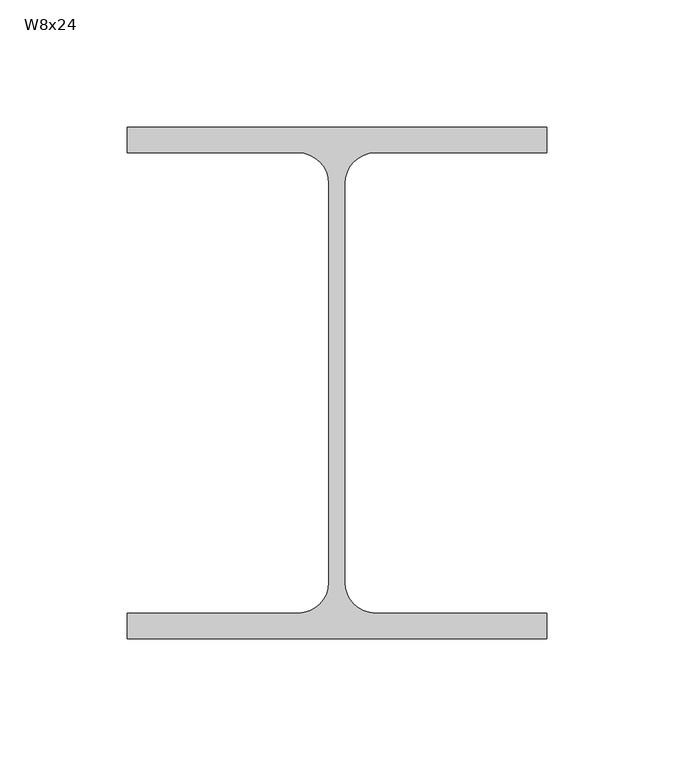
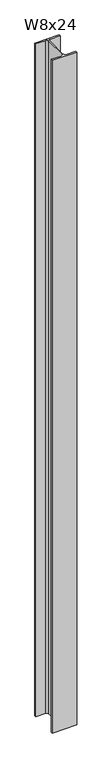
"""IFC4 building model written with IfcOpenShell, lengths in millimetres: column geometry, RME WF - Column : W8x24."""

from ifc_helpers import new_model, si_unit, point, frame, frame_2d, origin, place, context, project, spatial, polyline, circle_curve, trimmed, segment, composite_curve, outline, extrude, source, transform, mapped, element, save


def w8x24_d83c1f9c(model_context):
    return source(origin(), model_context, "Body", "SweptSolid", [
        extrude(outline(composite_curve([segment(polyline([(82.55, 100.711), (82.55, 90.551), (15.1765, 90.551)]), True, "CONTINUOUS"), segment(trimmed(circle_curve(frame_2d((15.1765, 78.486)), 12.065), [point((15.1765, 90.551))], [point((3.1115, 78.486))], True, "CARTESIAN"), True, "CONTINUOUS"), segment(polyline([(3.1115, 78.486), (3.1115, -78.486)]), True, "CONTINUOUS"), segment(trimmed(circle_curve(frame_2d((15.1765, -78.486)), 12.065), [point((3.1115, -78.486))], [point((15.1765, -90.551))], True, "CARTESIAN"), True, "CONTINUOUS"), segment(polyline([(15.1765, -90.551), (82.55, -90.551), (82.55, -100.711), (-82.55, -100.711), (-82.55, -90.551), (-15.1765, -90.551)]), True, "CONTINUOUS"), segment(trimmed(circle_curve(frame_2d((-15.1765, -78.486)), 12.065), [point((-15.1765, -90.551))], [point((-3.1115, -78.486))], True, "CARTESIAN"), True, "CONTINUOUS"), segment(polyline([(-3.1115, -78.486), (-3.1115, 78.486)]), True, "CONTINUOUS"), segment(trimmed(circle_curve(frame_2d((-15.1765, 78.486)), 12.065), [point((-3.1115, 78.486))], [point((-15.1765, 90.551))], True, "CARTESIAN"), True, "CONTINUOUS"), segment(polyline([(-15.1765, 90.551), (-82.55, 90.551), (-82.55, 100.711), (82.55, 100.711)]), True, "CONTINUOUS")], self_intersect=False)), frame((0.0, 0.0, -304.8), z_axis=(0.0, 0.0, 1.0), x_axis=(1.0, 0.0, 0.0)), (0.0, 0.0, 1.0), 4791.075),
    ])


if __name__ == "__main__":
    model = new_model("IFC4")
    model_context = context("Model", 3, world=origin())
    ifc_project = project(units=[si_unit("LENGTHUNIT", "METRE", prefix="MILLI")], contexts=[model_context])
    site = spatial("IfcSite", under=ifc_project)
    building = spatial("IfcBuilding", under=site)
    placement = place(None, origin())
    w8x24_shape = w8x24_d83c1f9c(model_context)
    element("IfcColumn", 1, ObjectType="RME WF - Column : W8x24", at=placement, inside=building, context=model_context, shape_type="MappedRepresentation", body=[
        mapped(w8x24_shape, transform((0.0, 0.0, 0.0), x_axis=(1.0, 0.0, 0.0), y_axis=(0.0, 1.0, 0.0), z_axis=(0.0, 0.0, 1.0))),
    ])
    save(model, "model.ifc")

# Revit data of these elements
# Type "RME WF - Column : W8x24"
#   Type Mark = "C1"
#   REINF TYPE [instance default] = ""
#   Nominal Size = "W16"
#   COL REMARKS [instance default] = ""
#   BP [instance default] = ""
#   Assembly Code = "B10"
#   W = 24
#   bf = 0' - 6 1/2"
#   d = 0' - 7.93"
#   k = 0' - 0 7/8"
#   kr = 0' - 0.475"
#   tf = 0' - 0.4"
#   tw = 0' - 0.245"
#   A = 0.0491667 SF
#   Structural Material [instance default] = Metal - Steel - ASTM A992
# Element 1 (IfcColumn, "RME WF - Column : W8x24")
#   Materials on its faces: "Metal - Steel - ASTM A992"
# Materials
#   "Metal - Steel - ASTM A992": class "Metal", colour RGB 255 128 0, transparency 0
